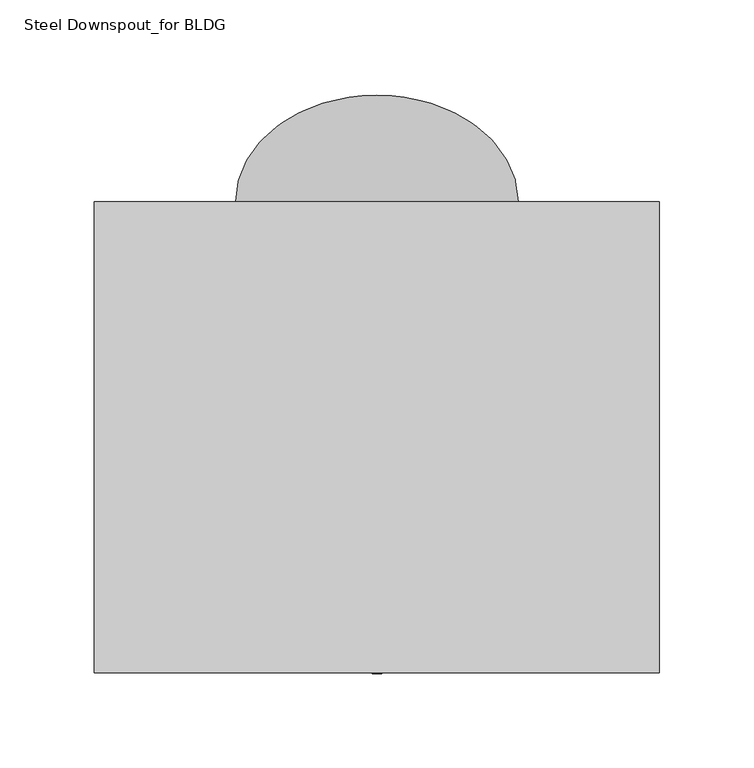
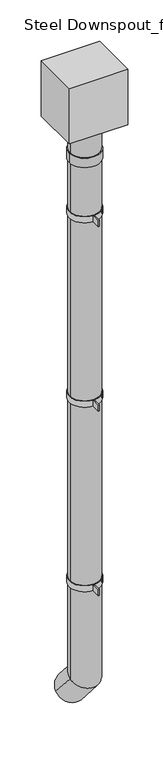
"""IFC4 building model written with IfcOpenShell, lengths in millimetres: proxy geometry, Steel Downspout_for BLDG : H_GM_AR_B07_Steel Downspout_D150."""

from ifc_helpers import new_model, si_unit, point, frame, origin, origin_with_axes, origin_2d, place, context, project, spatial, polyline, circle_curve, ellipse_curve, trimmed, segment, composite_curve, outline, extrude, source, transform, mapped, element, save
from ifc_brep_helpers import plane_surface, cylinder_surface, revolved_surface, advanced_brep


def steel_downspout_for_bldg_01f6fcb7(model_context):
    return source(origin(), model_context, "Body", "SolidModel", [
        extrude(outline(polyline([(2.5, -125.0), (-2.5, -125.0), (-2.5, -50.0), (2.5, -50.0), (2.5, -125.0)])), frame((0.0, 0.0, -500.0), z_axis=(0.0, 0.0, 1.0), x_axis=(1.0, 0.0, 0.0)), (0.0, 0.0, 1.0), 32.0),
        extrude(outline(composite_curve([segment(trimmed(circle_curve(origin_2d(), 80.0), [point((0.0, 80.0))], [point((0.0, -80.0))], False, "CARTESIAN"), True, "CONTINUOUS"), segment(trimmed(circle_curve(origin_2d(), 80.0), [point((0.0, -80.0))], [point((0.0, 80.0))], False, "CARTESIAN"), True, "CONTINUOUS")], self_intersect=False), holes=[composite_curve([segment(trimmed(circle_curve(origin_2d(), 75.0), [point((0.0, 75.0))], [point((0.0, -75.0))], True, "CARTESIAN"), True, "CONTINUOUS"), segment(trimmed(circle_curve(origin_2d(), 75.0), [point((0.0, -75.0))], [point((0.0, 75.0))], True, "CARTESIAN"), True, "CONTINUOUS")], self_intersect=False)]), frame((0.0, 0.0, -500.0), z_axis=(0.0, 0.0, 1.0), x_axis=(1.0, 0.0, 0.0)), (0.0, 0.0, 1.0), 32.0),
        extrude(outline(polyline([(2.5, -125.0), (-2.5, -125.0), (-2.5, -50.0), (2.5, -50.0), (2.5, -125.0)])), frame((0.0, 0.0, -1500.0), z_axis=(0.0, 0.0, 1.0), x_axis=(1.0, 0.0, 0.0)), (0.0, 0.0, 1.0), 32.0),
        extrude(outline(composite_curve([segment(trimmed(circle_curve(origin_2d(), 80.0), [point((0.0, 80.0))], [point((0.0, -80.0))], False, "CARTESIAN"), True, "CONTINUOUS"), segment(trimmed(circle_curve(origin_2d(), 80.0), [point((0.0, -80.0))], [point((0.0, 80.0))], False, "CARTESIAN"), True, "CONTINUOUS")], self_intersect=False), holes=[composite_curve([segment(trimmed(circle_curve(origin_2d(), 75.0), [point((0.0, 75.0))], [point((0.0, -75.0))], True, "CARTESIAN"), True, "CONTINUOUS"), segment(trimmed(circle_curve(origin_2d(), 75.0), [point((0.0, -75.0))], [point((0.0, 75.0))], True, "CARTESIAN"), True, "CONTINUOUS")], self_intersect=False)]), frame((0.0, 0.0, -1500.0), z_axis=(0.0, 0.0, 1.0), x_axis=(1.0, 0.0, 0.0)), (0.0, 0.0, 1.0), 32.0),
        advanced_brep(
        [(-75.0, 0.0, -200.0), (75.0, 0.0, -200.0), (-65.0, 0.0, -200.0), (65.0, 0.0, -200.0), (-65.0, 0.0, -3000.0), (65.0, 0.0, -3000.0), (-75.0, 0.0, -3000.0), (75.0, 0.0, -3000.0), (-75.0, 125.386264, -3144.2403969), (75.0, 125.386264, -3144.2403969), (-65.0, 125.386264, -3144.2403969), (65.0, 125.386264, -3144.2403969)],
        [
            (0, 1, circle_curve(frame((0.0, 0.0, -200.0), z_axis=(0.0, 0.0, 1.0), x_axis=(1.0, 0.0, 0.0)), 75.0)),
            (1, 0, circle_curve(frame((0.0, 0.0, -200.0), z_axis=(0.0, 0.0, 1.0), x_axis=(1.0, 0.0, 0.0)), 75.0)),
            (2, 3, circle_curve(frame((0.0, 0.0, -200.0), z_axis=(0.0, 0.0, -1.0), x_axis=(1.0, 0.0, 0.0)), 65.0)),
            (3, 2, circle_curve(frame((0.0, 0.0, -200.0), z_axis=(0.0, 0.0, -1.0), x_axis=(1.0, 0.0, 0.0)), 65.0)),
            (2, 4),
            (4, 5, ellipse_curve(frame((0.0, 0.0, -3000.0), z_axis=(0.0, 0.35020738125938633, -0.9366721892484279), x_axis=(0.0, -0.9366721892484279, -0.3502073812593867)), 69.3946086, 65.0)),
            (5, 3),
            (5, 4, ellipse_curve(frame((0.0, 0.0, -3000.0), z_axis=(0.0, 0.35020738125938633, -0.9366721892484279), x_axis=(0.0, -0.9366721892484279, -0.3502073812593867)), 69.3946086, 65.0)),
            (0, 6),
            (6, 7, ellipse_curve(frame((0.0, 0.0, -3000.0), z_axis=(0.0, -0.35020738125938633, 0.9366721892484279), x_axis=(0.0, 0.9366721892484279, 0.3502073812593867)), 80.0707023, 75.0)),
            (7, 1),
            (7, 6, ellipse_curve(frame((0.0, 0.0, -3000.0), z_axis=(0.0, -0.35020738125938633, 0.9366721892484279), x_axis=(0.0, 0.9366721892484279, 0.3502073812593867)), 80.0707023, 75.0)),
            (8, 9, circle_curve(frame((0.0, 125.386264, -3144.2403969), z_axis=(0.0, 0.6560590289903766, -0.7547095802228856), x_axis=(1.0, 0.0, 0.0)), 75.0)),
            (9, 8, circle_curve(frame((0.0, 125.386264, -3144.2403969), z_axis=(0.0, 0.6560590289903766, -0.7547095802228856), x_axis=(1.0, 0.0, 0.0)), 75.0)),
            (10, 11, circle_curve(frame((0.0, 125.386264, -3144.2403969), z_axis=(0.0, -0.6560590289903766, 0.7547095802228856), x_axis=(1.0, 0.0, 0.0)), 65.0)),
            (11, 10, circle_curve(frame((0.0, 125.386264, -3144.2403969), z_axis=(0.0, -0.6560590289903766, 0.7547095802228856), x_axis=(1.0, 0.0, 0.0)), 65.0)),
            (4, 10),
            (11, 5),
            (6, 8),
            (9, 7),
        ],
        [
            plane_surface(frame((0.0, 0.0, -200.0), z_axis=(0.0, 0.0, 1.0), x_axis=(1.0, 0.0, 0.0))),
            revolved_surface(polyline([(65.0, 0.0, -3024.302504151326), (65.0, 0.0, -200.0)]), (0.0, 0.0, -200.0), (0.0, 0.0, -1.0)),
            cylinder_surface(frame((0.0, 0.0, -200.0), z_axis=(0.0, 0.0, 1.0), x_axis=(1.0, 0.0, 0.0)), 75.0),
            plane_surface(frame((0.0, 125.386264, -3144.2403969), z_axis=(0.0, 0.6560590289903766, -0.7547095802228856), x_axis=(1.0, 0.0, 0.0))),
            revolved_surface(polyline([(65.0, 125.38626404697669, -3144.240396859164), (65.0, -15.943877275553579, -2981.6586672935878)]), (0.0, 0.0, -3000.0), (0.0, 0.6560590289903766, -0.7547095802228856)),
            cylinder_surface(frame((0.0, 0.0, -3000.0), z_axis=(0.0, -0.6560590289903766, 0.7547095802228856), x_axis=(1.0, 0.0, 0.0)), 75.0),
        ],
        [
            (0, [[1, 2], [3, 4]]),
            (1, [[-3, 5, 6, 7]]),
            (1, [[-4, -7, 8, -5]]),
            (2, [[-1, 9, 10, 11]]),
            (2, [[-2, -11, 12, -9]]),
            (3, [[13, 14], [15, 16]]),
            (4, [[-6, 17, -16, 18]]),
            (4, [[-8, -18, -15, -17]]),
            (5, [[-10, 19, -14, 20]]),
            (5, [[-12, -20, -13, -19]]),
        ],
    ),
        extrude(outline(polyline([(150.0, 125.0), (150.0, -125.0), (-150.0, -125.0), (-150.0, 125.0), (150.0, 125.0)])), origin_with_axes(), (0.0, 0.0, 1.0), 300.0),
        extrude(outline(polyline([(2.5, -125.0), (-2.5, -125.0), (-2.5, -50.0), (2.5, -50.0), (2.5, -125.0)])), frame((0.0, 0.0, -2500.0), z_axis=(0.0, 0.0, 1.0), x_axis=(1.0, 0.0, 0.0)), (0.0, 0.0, 1.0), 32.0),
        extrude(outline(composite_curve([segment(trimmed(circle_curve(origin_2d(), 80.0), [point((0.0, 80.0))], [point((0.0, -80.0))], False, "CARTESIAN"), True, "CONTINUOUS"), segment(trimmed(circle_curve(origin_2d(), 80.0), [point((0.0, -80.0))], [point((0.0, 80.0))], False, "CARTESIAN"), True, "CONTINUOUS")], self_intersect=False), holes=[composite_curve([segment(trimmed(circle_curve(origin_2d(), 75.0), [point((0.0, 75.0))], [point((0.0, -75.0))], True, "CARTESIAN"), True, "CONTINUOUS"), segment(trimmed(circle_curve(origin_2d(), 75.0), [point((0.0, -75.0))], [point((0.0, 75.0))], True, "CARTESIAN"), True, "CONTINUOUS")], self_intersect=False)]), frame((0.0, 0.0, -2500.0), z_axis=(0.0, 0.0, 1.0), x_axis=(1.0, 0.0, 0.0)), (0.0, 0.0, 1.0), 32.0),
        extrude(outline(composite_curve([segment(trimmed(circle_curve(origin_2d(), 80.0), [point((-80.0, 0.0))], [point((80.0, 0.0))], False, "CARTESIAN"), True, "CONTINUOUS"), segment(trimmed(circle_curve(origin_2d(), 80.0), [point((80.0, 0.0))], [point((-80.0, 0.0))], False, "CARTESIAN"), True, "CONTINUOUS")], self_intersect=False), holes=[composite_curve([segment(trimmed(circle_curve(origin_2d(), 65.0), [point((-65.0, 0.0))], [point((65.0, 0.0))], True, "CARTESIAN"), True, "CONTINUOUS"), segment(trimmed(circle_curve(origin_2d(), 65.0), [point((65.0, 0.0))], [point((-65.0, 0.0))], True, "CARTESIAN"), True, "CONTINUOUS")], self_intersect=False)]), frame((0.0, 0.0, -200.0), z_axis=(0.0, 0.0, 1.0), x_axis=(1.0, 0.0, 0.0)), (0.0, 0.0, 1.0), 50.0),
        extrude(outline(composite_curve([segment(trimmed(circle_curve(origin_2d(), 75.0), [point((-75.0, 0.0))], [point((75.0, 0.0))], False, "CARTESIAN"), True, "CONTINUOUS"), segment(trimmed(circle_curve(origin_2d(), 75.0), [point((75.0, 0.0))], [point((-75.0, 0.0))], False, "CARTESIAN"), True, "CONTINUOUS")], self_intersect=False), holes=[composite_curve([segment(trimmed(circle_curve(origin_2d(), 65.0), [point((-65.0, 0.0))], [point((65.0, 0.0))], True, "CARTESIAN"), True, "CONTINUOUS"), segment(trimmed(circle_curve(origin_2d(), 65.0), [point((65.0, 0.0))], [point((-65.0, 0.0))], True, "CARTESIAN"), True, "CONTINUOUS")], self_intersect=False)]), frame((0.0, 0.0, -150.0), z_axis=(0.0, 0.0, 1.0), x_axis=(1.0, 0.0, 0.0)), (0.0, 0.0, 1.0), 150.0),
    ])


if __name__ == "__main__":
    model = new_model("IFC4")
    model_context = context("Model", 3, world=origin())
    ifc_project = project(units=[si_unit("LENGTHUNIT", "METRE", prefix="MILLI")], contexts=[model_context])
    site = spatial("IfcSite", under=ifc_project)
    building = spatial("IfcBuilding", under=site)
    placement = place(None, origin())
    steel_downspout_for_bldg_shape = steel_downspout_for_bldg_01f6fcb7(model_context)
    element("IfcBuildingElementProxy", 1, Name="Steel Downspout_for BLDG : H_GM_AR_B07_Steel Downspout_D150", ObjectType="Steel Downspout_for BLDG : H_GM_AR_B07_Steel Downspout_D150", at=placement, inside=building, context=model_context, shape_type="MappedRepresentation", body=[
        mapped(steel_downspout_for_bldg_shape, transform((0.0, 0.0, 0.0), x_axis=(1.0, 0.0, 0.0), y_axis=(0.0, 1.0, 0.0), z_axis=(0.0, 0.0, 1.0))),
    ])
    save(model, "model.ifc")

# Revit data of these elements
# Type "Steel Downspout_for BLDG : H_GM_AR_B07_Steel Downspout_D150"
#   외벽 거리 = 100 mm
#   Rainwater Downpipe Height [instance default] = 15056 mm
#   H [instance default] = 15056 mm
#   r_int. = 65 mm
#   r_bold = 80 mm
#   r = 75 mm
#   D = 150 mm
#   Box Width = 300 mm
#   Box Length = 250 mm
#   Box Height = 300 mm
#   EA [instance default] = 15
#   Material_Name = 00_Metal_Steel
#   Default Elevation = 0
# Element 1 (IfcBuildingElementProxy, "Steel Downspout_for BLDG : H_GM_AR_B07_Steel Downspout_D150")
#   Rainwater Downpipe Height = 3000 mm
#   H = 3000 mm
#   EA = 3
#   Materials on its faces: "00_Metal_Steel"
# Materials
#   "00_Metal_Steel": class "Metal", colour RGB 148 148 148, transparency 0, Description = "Steel", Cost = 0, Image = Doors - Windows.Glazed Curtain Walls.Stainless Steel Curtain Wall.jpg
